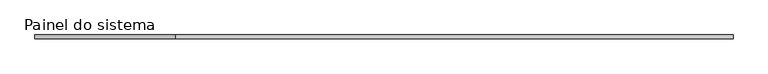
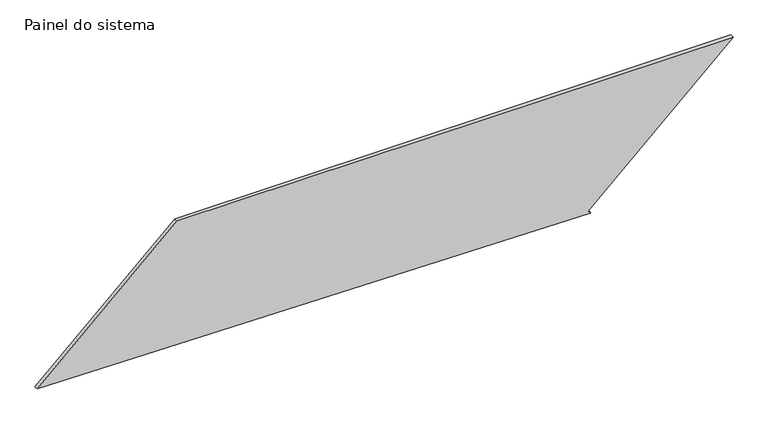
"""IFC4 building model written with IfcOpenShell, lengths in millimetres: plate geometry, Painel do sistema : Envidraçado."""

from ifc_helpers import new_model, si_unit, frame, origin, place, context, project, spatial, polyline, outline, extrude, source, transform, mapped, element, save


def painel_do_sistema_f999112a(model_context):
    return source(origin(), model_context, "Body", "SweptSolid", [
        extrude(outline(polyline([(0.0, 1389.3611285), (18.3764951, 1372.4110717), (920.4718928, 2350.4226407), (920.4718928, -1407.1295872), (50.400056, -2350.4226407), (0.0, 1389.3611285)])), frame((0.0, 24.5, 0.0), z_axis=(0.0, 1.0, 0.0), x_axis=(0.0, 0.0, 1.0)), (0.0, 0.0, 1.0), 25.0),
    ])


if __name__ == "__main__":
    model = new_model("IFC4")
    model_context = context("Model", 3, world=origin())
    ifc_project = project(units=[si_unit("LENGTHUNIT", "METRE", prefix="MILLI")], contexts=[model_context])
    site = spatial("IfcSite", under=ifc_project)
    building = spatial("IfcBuilding", under=site)
    placement = place(None, origin())
    painel_do_sistema_shape = painel_do_sistema_f999112a(model_context)
    element("IfcPlate", 1, ObjectType="Painel do sistema : Envidraçado", at=placement, inside=building, context=model_context, shape_type="MappedRepresentation", body=[
        mapped(painel_do_sistema_shape, transform((0.0, 0.0, 0.0), x_axis=(1.0, 0.0, 0.0), y_axis=(0.0, 1.0, 0.0), z_axis=(0.0, 0.0, 1.0))),
    ])
    save(model, "model.ifc")

# Revit data of these elements
# Type "Painel do sistema : Envidraçado"
#   Construction Type Id = "GSP4R"
#   Analytic Construction = "Vidraça única Pilkington 1/8 pol"
#   Visual Light Transmittance = 0.9
#   Solar Heat Gain Coefficient = 0.86
#   Heat Transfer Coefficient (U) = 6.7069 W/(m²·K)
# Element 1 (IfcPlate, "Painel do sistema : Envidraçado")
#   Materials on its faces: "Vidro"
# Materials
#   "Vidro": class "Vidro", colour RGB 0 128 192, transparency 0.9, Description = "Vidro de sílica", Cost = 0
